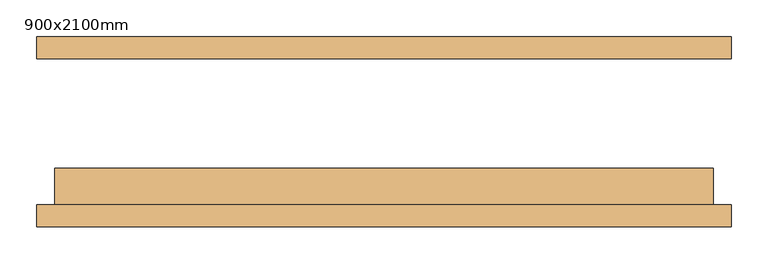
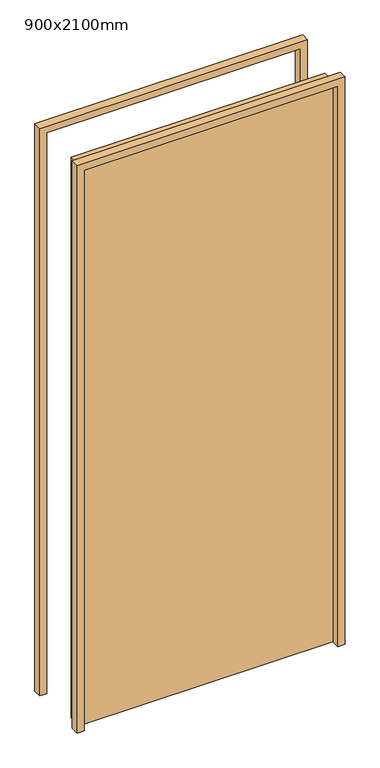
"""IFC4 building model written with IfcOpenShell, lengths in millimetres: door geometry, WWm-SingleSolid-Flush : 900x2100mm."""

from ifc_helpers import new_model, si_unit, frame, origin, origin_with_axes, place, context, project, spatial, polyline, outline, extrude, source, transform, mapped, element, save


def door_900x2100mm_9b55c49e(model_context):
    return source(origin(), model_context, "Body", "SweptSolid", [
        extrude(outline(polyline([(2125.0, -475.0), (0.0, -475.0), (0.0, -450.0), (2100.0, -450.0), (2100.0, 450.0), (0.0, 450.0), (0.0, 475.0), (2125.0, 475.0), (2125.0, -475.0)])), frame((0.0, -130.0, 0.0), z_axis=(0.0, 1.0, 0.0), x_axis=(0.0, 0.0, 1.0)), (0.0, 0.0, 1.0), 30.0),
        extrude(outline(polyline([(2125.0, 475.0), (2125.0, -475.0), (0.0, -475.0), (0.0, -450.0), (2100.0, -450.0), (2100.0, 450.0), (0.0, 450.0), (0.0, 475.0), (2125.0, 475.0)])), frame((0.0, 100.0, 0.0), z_axis=(0.0, 1.0, 0.0), x_axis=(0.0, 0.0, 1.0)), (0.0, 0.0, 1.0), 30.0),
        extrude(outline(polyline([(450.0, -50.0), (450.0, -100.0), (-450.0, -100.0), (-450.0, -50.0), (450.0, -50.0)])), origin_with_axes(), (0.0, 0.0, 1.0), 2100.0),
    ])


if __name__ == "__main__":
    model = new_model("IFC4")
    model_context = context("Model", 3, world=origin())
    ifc_project = project(units=[si_unit("LENGTHUNIT", "METRE", prefix="MILLI")], contexts=[model_context])
    site = spatial("IfcSite", under=ifc_project)
    building = spatial("IfcBuilding", under=site)
    placement = place(None, origin())
    door_900x2100mm_shape = door_900x2100mm_9b55c49e(model_context)
    element("IfcDoor", 1, ObjectType="WWm-SingleSolid-Flush : 900x2100mm", at=placement, inside=building, context=model_context, shape_type="MappedRepresentation", body=[
        mapped(door_900x2100mm_shape, transform((0.0, 0.0, 0.0), x_axis=(1.0, 0.0, 0.0), y_axis=(0.0, 1.0, 0.0), z_axis=(0.0, 0.0, 1.0))),
    ])
    save(model, "model.ifc")

# Revit data of these elements
# Type "WWm-SingleSolid-Flush : 900x2100mm"
#   Type Mark = "EX1-52"
#   Construction Type Id = "MDOOR"
#   Assembly Code = "C1020"
#   Analytic Construction = "Metal"
#   Thickness = 50 mm
#   Thermal Resistance (R) = 0.270117 (m²·K)/W
#   Heat Transfer Coefficient (U) = 3.7021 W/(m²·K)
#   Height = 2100 mm
#   Trim Projection Ext = 30 mm
#   Trim Projection Int = 30 mm
#   Trim Width = 25 mm
#   Width = 900 mm
#   Not 90 Degree [instance default] = no
#   90 Degree [instance default] = yes
#   Door Material = WW-EC-RGB-White
#   Frame Material = WW-EC-RGB-White
#   Visual Light Transmittance = 0
#   Solar Heat Gain Coefficient = 0
#   Function = (empty or 0)
#   Wall Closure = (empty or 0)
# Element 1 (IfcDoor, "WWm-SingleSolid-Flush : 900x2100mm")
#   Materials on its faces: "WW-EC-RGB-White"
# Materials
#   "WW-EC-RGB-White": class "Generic", colour RGB 255 255 255, transparency 0, Comments = "If region requests off-white, swith asset color to RGB 231-228-220", Description = "Generic Color", Cost = 0
